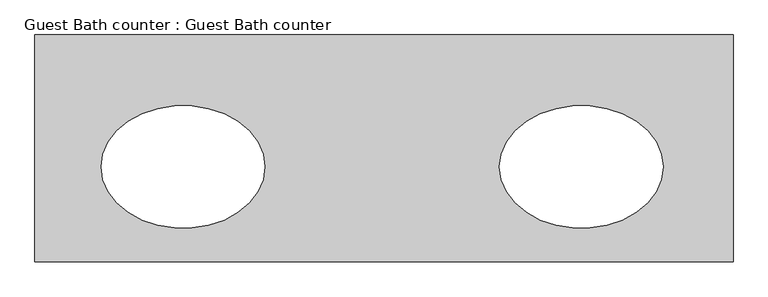
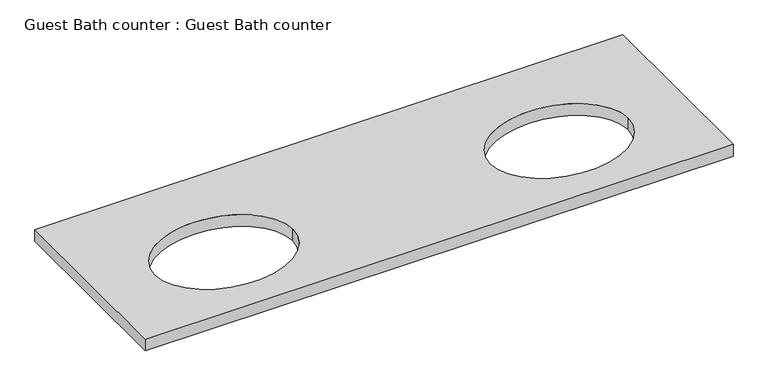
"""IFC4 building model written with IfcOpenShell, lengths in millimetres: furniture geometry, Guest Bath counter : Guest Bath counter."""

from ifc_helpers import new_model, si_unit, point, frame, origin, place, context, project, spatial, ellipse_curve, trimmed, source, transform, mapped, element, save
from ifc_brep_helpers import plane_surface, extruded_surface, advanced_brep


def guest_bath_counter_guest_bath_counter_5d591adb(model_context):
    return source(origin(), model_context, "Body", "AdvancedBrep", [
        advanced_brep(
        [(8469.3125, 12897.64375, 3905.25), (10275.8875, 12897.64375, 3905.25), (10275.8875, 13484.2034596, 3905.25), (8469.3125, 13484.2034596, 3905.25), (9064.6737671, 13142.7582521, 3905.25), (8640.6737671, 13142.7582521, 3905.25), (10095.2570391, 13142.7582521, 3905.25), (9671.2570391, 13142.7582521, 3905.25), (8469.3125, 12897.64375, 3867.15), (8469.3125, 13484.2034596, 3867.15), (10275.8875, 13484.2034596, 3867.15), (10275.8875, 12897.64375, 3867.15), (9064.6737671, 13142.7582521, 3867.15), (8640.6737671, 13142.7582521, 3867.15), (10095.2570391, 13142.7582521, 3867.15), (9671.2570391, 13142.7582521, 3867.15)],
        [
            (0, 1),
            (1, 2),
            (2, 3),
            (3, 0),
            (4, 5, ellipse_curve(frame((8852.6737671, 13142.7582521, 3905.25), z_axis=(0.0, 0.0, -1.0), x_axis=(-1.0, 0.0, 0.0)), 212.0, 158.7697221)),
            (5, 4, ellipse_curve(frame((8852.6737671, 13142.7582521, 3905.25), z_axis=(0.0, 0.0, -1.0), x_axis=(-1.0, 0.0, 0.0)), 212.0, 158.7697221)),
            (6, 7, ellipse_curve(frame((9883.2570391, 13142.7582521, 3905.25), z_axis=(0.0, 0.0, -1.0), x_axis=(-1.0, 0.0, 0.0)), 212.0, 158.7697221)),
            (7, 6, ellipse_curve(frame((9883.2570391, 13142.7582521, 3905.25), z_axis=(0.0, 0.0, -1.0), x_axis=(-1.0, 0.0, 0.0)), 212.0, 158.7697221)),
            (8, 9),
            (9, 10),
            (10, 11),
            (11, 8),
            (12, 13, ellipse_curve(frame((8852.6737671, 13142.7582521, 3867.15), z_axis=(0.0, 0.0, 1.0), x_axis=(-1.0, 0.0, 0.0)), 212.0, 158.7697221)),
            (13, 12, ellipse_curve(frame((8852.6737671, 13142.7582521, 3867.15), z_axis=(0.0, 0.0, 1.0), x_axis=(-1.0, 0.0, 0.0)), 212.0, 158.7697221)),
            (14, 15, ellipse_curve(frame((9883.2570391, 13142.7582521, 3867.15), z_axis=(0.0, 0.0, 1.0), x_axis=(-1.0, 0.0, 0.0)), 212.0, 158.7697221)),
            (15, 14, ellipse_curve(frame((9883.2570391, 13142.7582521, 3867.15), z_axis=(0.0, 0.0, 1.0), x_axis=(-1.0, 0.0, 0.0)), 212.0, 158.7697221)),
            (0, 8),
            (11, 1),
            (10, 2),
            (9, 3),
            (4, 12),
            (13, 5),
            (6, 14),
            (15, 7),
        ],
        [
            plane_surface(frame((8509.0, 12897.64375, 3905.25), z_axis=(0.0, 0.0, 1.0), x_axis=(1.0, 0.0, 0.0))),
            plane_surface(frame((8509.0, 12897.64375, 3867.15), z_axis=(0.0, 0.0, -1.0), x_axis=(-1.0, 0.0, 0.0))),
            plane_surface(frame((8469.3125, 12897.64375, 3905.25), z_axis=(0.0, -1.0, 0.0), x_axis=(0.0, 0.0, -1.0))),
            plane_surface(frame((10275.8875, 12897.64375, 3905.25), z_axis=(1.0, 0.0, 0.0), x_axis=(0.0, 0.0, -1.0))),
            plane_surface(frame((10275.8875, 13484.2034596, 3905.25), z_axis=(0.0, 1.0, 0.0), x_axis=(0.0, 0.0, -1.0))),
            plane_surface(frame((8469.3125, 13484.2034596, 3905.25), z_axis=(-1.0, 0.0, 0.0), x_axis=(0.0, 0.0, -1.0))),
            extruded_surface(trimmed(ellipse_curve(frame((8852.6737671, 13142.7582521, 3028.95), z_axis=(0.0, 0.0, -1.0), x_axis=(-1.0, 0.0, 0.0)), 212.0, 158.7697221), [point((9064.6737671, 13142.7582521, 3028.95))], [point((8640.6737671, 13142.7582521, 3028.95))], True, "CARTESIAN"), (0.0, 0.0, 38.100000000000364), 38.100000000000364),
            extruded_surface(trimmed(ellipse_curve(frame((8852.6737671, 13142.7582521, 3028.95), z_axis=(0.0, 0.0, -1.0), x_axis=(-1.0, 0.0, 0.0)), 212.0, 158.7697221), [point((8640.6737671, 13142.7582521, 3028.95))], [point((9064.6737671, 13142.7582521, 3028.95))], True, "CARTESIAN"), (0.0, 0.0, 38.100000000000364), 38.100000000000364),
            extruded_surface(trimmed(ellipse_curve(frame((9883.2570391, 13142.7582521, 3028.95), z_axis=(0.0, 0.0, -1.0), x_axis=(-1.0, 0.0, 0.0)), 212.0, 158.7697221), [point((10095.2570391, 13142.7582521, 3028.95))], [point((9671.2570391, 13142.7582521, 3028.95))], True, "CARTESIAN"), (0.0, 0.0, 38.100000000000364), 38.100000000000364),
            extruded_surface(trimmed(ellipse_curve(frame((9883.2570391, 13142.7582521, 3028.95), z_axis=(0.0, 0.0, -1.0), x_axis=(-1.0, 0.0, 0.0)), 212.0, 158.7697221), [point((9671.2570391, 13142.7582521, 3028.95))], [point((10095.2570391, 13142.7582521, 3028.95))], True, "CARTESIAN"), (0.0, 0.0, 38.100000000000364), 38.100000000000364),
        ],
        [
            (0, [[1, 2, 3, 4], [5, 6], [7, 8]]),
            (1, [[9, 10, 11, 12], [13, 14], [15, 16]]),
            (2, [[-1, 17, -12, 18]]),
            (3, [[-2, -18, -11, 19]]),
            (4, [[-3, -19, -10, 20]]),
            (5, [[-4, -20, -9, -17]]),
            (6, [[-5, 21, -14, 22]]),
            (7, [[-6, -22, -13, -21]]),
            (8, [[-7, 23, -16, 24]]),
            (9, [[-8, -24, -15, -23]]),
        ],
    ),
    ])


if __name__ == "__main__":
    model = new_model("IFC4")
    model_context = context("Model", 3, world=origin())
    ifc_project = project(units=[si_unit("LENGTHUNIT", "METRE", prefix="MILLI")], contexts=[model_context])
    site = spatial("IfcSite", under=ifc_project)
    building = spatial("IfcBuilding", under=site)
    placement = place(None, origin())
    guest_bath_counter_guest_bath_counter_shape = guest_bath_counter_guest_bath_counter_5d591adb(model_context)
    element("IfcFurniture", 1, ObjectType="Guest Bath counter : Guest Bath counter", at=placement, inside=building, context=model_context, shape_type="MappedRepresentation", body=[
        mapped(guest_bath_counter_guest_bath_counter_shape, transform((0.0, 0.0, 0.0), x_axis=(1.0, 0.0, 0.0), y_axis=(0.0, 1.0, 0.0), z_axis=(0.0, 0.0, 1.0))),
    ])
    save(model, "model.ifc")

# Revit data of these elements
# Type "Guest Bath counter : Guest Bath counter"
#   COBie.Type = no
# Element 1 (IfcFurniture, "Guest Bath counter : Guest Bath counter")
#   Materials on its faces: "Corian - Dusk"
# Materials
#   "Corian - Dusk": class "Plastic", colour RGB 75 95 146, transparency 0, Manufacturer = "Corning", Cost = 0
